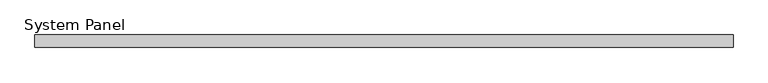
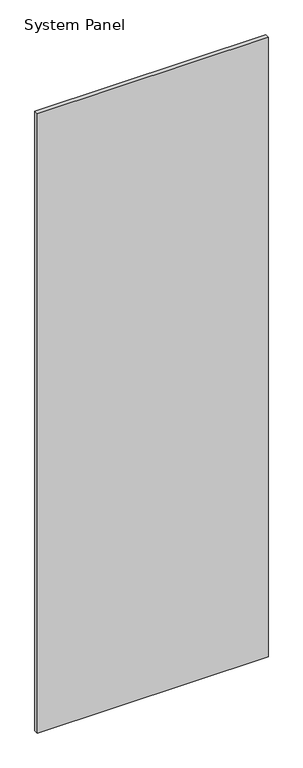
"""IFC4 building model written with IfcOpenShell, lengths in millimetres: plate geometry, System Panel : WWm-Glass-20mm-10mmOffset."""

import ifcopenshell
import ifcopenshell.guid

model = None  # the IFC model being written
_history = None  # IfcOwnerHistory: only IFC2X3 demands one
_inside = {}  # id of a spatial element -> (the spatial element, [elements in it])
_under = {}  # id of a project, library or spatial element -> (it, [spatial elements below it])
_declared = {}  # id of a project -> (the project, [libraries it declares])
_typed = {}  # id of a type object -> (the type object, [elements of that type])
_made_of = {}  # id of a material, layer set ... -> (it, [elements and type objects made of it])


def new_model(schema):
    """Start an empty IFC model of exactly this schema.

    Asked for "IFC4X3", IfcOpenShell would pick the latest addendum, in which some entities
    have other attributes; the version numbers below select the first issue.
    IFC2X3 requires an IfcOwnerHistory on every rooted entity: one is made here for all.
    """
    global model, _history
    if schema == "IFC4X3":
        model = ifcopenshell.file(schema_version=(4, 3, 0, 0))
    else:
        model = ifcopenshell.file(schema=schema)
    _inside.clear()
    _under.clear()
    _declared.clear()
    _typed.clear()
    _made_of.clear()
    _history = None
    if model.schema == "IFC2X3":
        org = make("IfcOrganization", Name="unknown")
        user = make(
            "IfcPersonAndOrganization",
            ThePerson=make("IfcPerson", FamilyName="unknown"),
            TheOrganization=org,
        )
        app = make(
            "IfcApplication",
            ApplicationDeveloper=org,
            Version="unknown",
            ApplicationFullName="unknown",
            ApplicationIdentifier="unknown",
        )
        _history = make(
            "IfcOwnerHistory",
            OwningUser=user,
            OwningApplication=app,
            ChangeAction="ADDED",
            CreationDate=0,
        )
    return model


def make(cls, **values):
    """One entity of the class cls with the attributes given. An attribute that is None is left unset."""
    return model.create_entity(
        cls, **{name: value for name, value in values.items() if value is not None}
    )


def rooted(cls, **values):
    """An entity with a GlobalId (a new one), such as an element, a storey or a relation."""
    return make(cls, GlobalId=ifcopenshell.guid.new(), OwnerHistory=_history, **values)


def si_unit(unit_type, name, prefix=None):
    """IfcSIUnit, for example si_unit("LENGTHUNIT", "METRE", prefix="MILLI")."""
    return make("IfcSIUnit", UnitType=unit_type, Prefix=prefix, Name=name)


def assignment(units):
    """IfcUnitAssignment: the units of a project."""
    return None if units is None else make("IfcUnitAssignment", Units=units)


def point(xyz):
    """IfcCartesianPoint."""
    return None if xyz is None else make("IfcCartesianPoint", Coordinates=xyz)


def direction(xyz):
    """IfcDirection."""
    return None if xyz is None else make("IfcDirection", DirectionRatios=xyz)


def frame(location, z_axis=None, x_axis=None):
    """IfcAxis2Placement3D, a coordinate frame: its origin and axes. An axis left out is left unset."""
    return make(
        "IfcAxis2Placement3D",
        Location=point(location),
        Axis=direction(z_axis),
        RefDirection=direction(x_axis),
    )


def origin():
    """The frame at (0, 0, 0) with its axes left unset."""
    return frame((0.0, 0.0, 0.0))


def origin_with_axes():
    """The frame at (0, 0, 0) with the z axis (0, 0, 1) and the x axis (1, 0, 0) written out."""
    return frame((0.0, 0.0, 0.0), z_axis=(0.0, 0.0, 1.0), x_axis=(1.0, 0.0, 0.0))


def place(relative_to, where):
    """IfcLocalPlacement: puts the frame where relative to a parent placement (None: the world)."""
    return make(
        "IfcLocalPlacement", PlacementRelTo=relative_to, RelativePlacement=where
    )


def context(
    kind, dimensions, precision=None, world=None, true_north=None, identifier=None
):
    """IfcGeometricRepresentationContext, for example the 3D "Model" context."""
    return make(
        "IfcGeometricRepresentationContext",
        ContextIdentifier=identifier,
        ContextType=kind,
        CoordinateSpaceDimension=dimensions,
        Precision=precision,
        WorldCoordinateSystem=world,
        TrueNorth=true_north,
    )


def project(units=None, contexts=None):
    """IfcProject with its units and contexts."""
    return rooted(
        "IfcProject",
        Name="project",
        RepresentationContexts=contexts,
        UnitsInContext=assignment(units),
    )


def spatial(cls, under=None, at=None, **own):
    """A site, building, storey or space (cls), placed at a placement, below another one or the project."""
    s = rooted(cls, ObjectPlacement=at, **own)
    if under is not None:
        _under.setdefault(under.id(), (under, []))[1].append(s)
    return s


def polyline(points):
    """IfcPolyline through the points."""
    return make("IfcPolyline", Points=[point(p) for p in points])


def outline(outer, holes=None, kind="AREA"):
    """IfcArbitraryClosedProfileDef: a profile drawn as a closed curve; with holes, ...WithVoids."""
    if holes is None:
        return make("IfcArbitraryClosedProfileDef", ProfileType=kind, OuterCurve=outer)
    return make(
        "IfcArbitraryProfileDefWithVoids",
        ProfileType=kind,
        OuterCurve=outer,
        InnerCurves=holes,
    )


def extrude(swept, where, along, depth):
    """IfcExtrudedAreaSolid: the profile swept, set in the frame where, extruded along a direction by depth."""
    return make(
        "IfcExtrudedAreaSolid",
        SweptArea=swept,
        Position=where,
        ExtrudedDirection=direction(along),
        Depth=depth,
    )


def shape(context_of_items, identifier, shape_type, items):
    """IfcShapeRepresentation: the items that make up one representation, for example the "Body"."""
    return make(
        "IfcShapeRepresentation",
        ContextOfItems=context_of_items,
        RepresentationIdentifier=identifier,
        RepresentationType=shape_type,
        Items=items,
    )


def source(mapping_origin, context_of_items, identifier, shape_type, items):
    """IfcRepresentationMap: a shape defined once, which mapped items show again and again."""
    return make(
        "IfcRepresentationMap",
        MappingOrigin=mapping_origin,
        MappedRepresentation=shape(context_of_items, identifier, shape_type, items),
    )


def transform(
    local_origin,
    x_axis=None,
    y_axis=None,
    z_axis=None,
    scale=None,
    scale2=None,
    scale3=None,
    uniform=True,
):
    """IfcCartesianTransformationOperator3D, or its non-uniform kind. x_axis, y_axis, z_axis: its Axis1, 2, 3."""
    if uniform:
        return make(
            "IfcCartesianTransformationOperator3D",
            Axis1=direction(x_axis),
            Axis2=direction(y_axis),
            LocalOrigin=point(local_origin),
            Scale=scale,
            Axis3=direction(z_axis),
        )
    return make(
        "IfcCartesianTransformationOperator3DnonUniform",
        Axis1=direction(x_axis),
        Axis2=direction(y_axis),
        LocalOrigin=point(local_origin),
        Scale=scale,
        Axis3=direction(z_axis),
        Scale2=scale2,
        Scale3=scale3,
    )


def mapped(mapping_source, mapping_target):
    """IfcMappedItem: shows the shape of a source again, moved by a transform."""
    return make(
        "IfcMappedItem", MappingSource=mapping_source, MappingTarget=mapping_target
    )


def made_of(thing, what):
    """Note that an element or type object is made of a material, layer set ...; save() writes the relation."""
    if what is not None:
        _made_of.setdefault(what.id(), (what, []))[1].append(thing)
    return thing


def element(
    cls,
    number,
    at=None,
    inside=None,
    cuts=None,
    type_object=None,
    material=None,
    context=None,
    identifier="Body",
    shape_type=None,
    held_by="IfcProductDefinitionShape",
    body=None,
    shapes=None,
    **own,
):
    """One element of the class cls, such as IfcWall. Its Tag is "e" and its number.

    at: its placement. inside: the storey or other place that contains it. cuts: it is an
    opening in that element (IfcRelVoidsElement). A single representation is given by context,
    identifier, shape_type and body (its items); several are given by shapes. held_by: the class
    of the entity that holds the representations. save() writes the other relations.
    """
    e = rooted(cls, Tag="e%d" % number, ObjectPlacement=at, **own)
    if body is not None:
        shapes = [shape(context, identifier, shape_type, body)]
    if shapes is not None:
        e.Representation = make(held_by, Representations=shapes)
    if inside is not None:
        _inside.setdefault(inside.id(), (inside, []))[1].append(e)
    if cuts is not None:
        rooted(
            "IfcRelVoidsElement", RelatingBuildingElement=cuts, RelatedOpeningElement=e
        )
    if type_object is not None:
        _typed.setdefault(type_object.id(), (type_object, []))[1].append(e)
    return made_of(e, material)


def aggregate(whole, parts):
    """IfcRelAggregates: a whole, such as a stair, and the parts it consists of."""
    return rooted("IfcRelAggregates", RelatingObject=whole, RelatedObjects=parts)


def save(model, path):
    """Write the relations noted so far, then the file.

    IfcRelAggregates (storeys below a building ...), IfcRelContainedInSpatialStructure (elements
    in a storey), IfcRelDefinesByType, IfcRelAssociatesMaterial and IfcRelDeclares: one each for
    every whole, place, type object, material and project.
    """
    for whole, parts in _under.values():
        aggregate(whole, parts)
    for where, things in _inside.values():
        rooted(
            "IfcRelContainedInSpatialStructure",
            RelatedElements=things,
            RelatingStructure=where,
        )
    for kind, things in _typed.values():
        rooted("IfcRelDefinesByType", RelatedObjects=things, RelatingType=kind)
    for what, things in _made_of.values():
        rooted("IfcRelAssociatesMaterial", RelatedObjects=things, RelatingMaterial=what)
    for by, libraries in _declared.values():
        rooted("IfcRelDeclares", RelatingContext=by, RelatedDefinitions=libraries)
    model.write(path)


def system_panel_6fd85a04(model_context):
    return source(origin(), model_context, "Body", "SweptSolid", [
        extrude(outline(polyline([(555.0, 0.0), (-555.0, 0.0), (-555.0, 20.0), (555.0, 20.0), (555.0, 0.0)])), origin_with_axes(), (0.0, 0.0, 1.0), 3150.0),
    ])


if __name__ == "__main__":
    model = new_model("IFC4")
    model_context = context("Model", 3, world=origin())
    ifc_project = project(units=[si_unit("LENGTHUNIT", "METRE", prefix="MILLI")], contexts=[model_context])
    site = spatial("IfcSite", under=ifc_project)
    building = spatial("IfcBuilding", under=site)
    placement = place(None, origin())
    system_panel_shape = system_panel_6fd85a04(model_context)
    element("IfcPlate", 1, ObjectType="System Panel : WWm-Glass-20mm-10mmOffset", at=placement, inside=building, context=model_context, shape_type="MappedRepresentation", body=[
        mapped(system_panel_shape, transform((0.0, 0.0, 0.0), x_axis=(1.0, 0.0, 0.0), y_axis=(0.0, 1.0, 0.0), z_axis=(0.0, 0.0, 1.0))),
    ])
    save(model, "model.ifc")

# Revit data of these elements
# Type "System Panel : WWm-Glass-20mm-10mmOffset"
#   Finish = ""
# Element 1 (IfcPlate, "System Panel : WWm-Glass-20mm-10mmOffset")
#   Materials on its faces: "WW-EC-GL-Storefront"
# Materials
#   "WW-EC-GL-Storefront": class "Glass", colour RGB 236 240 239, transparency 0.85, Description = "Storefront Glass", Cost = 0
